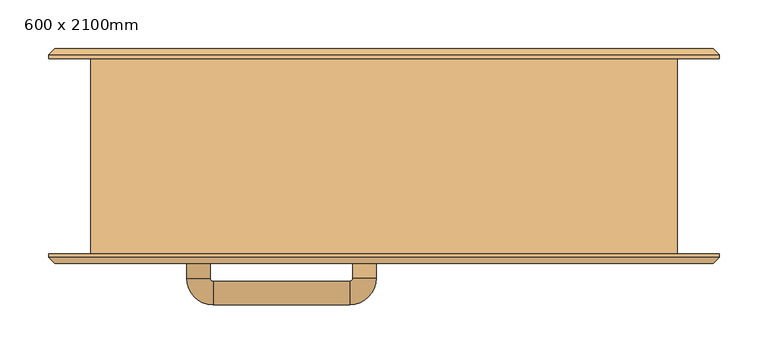
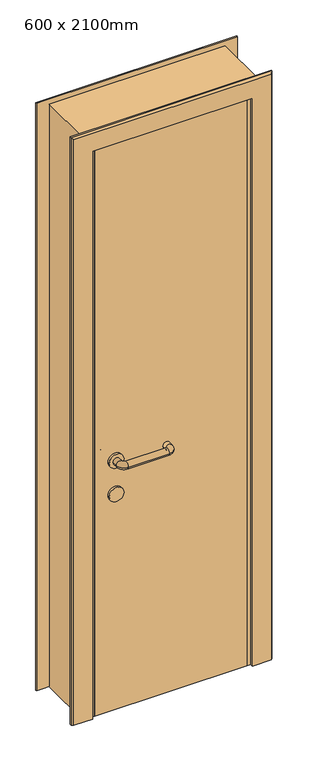
"""IFC4 building model written with IfcOpenShell, lengths in millimetres: door geometry, Porta única com revestimento : 600 x 2100mm."""

from ifc_helpers import new_model, si_unit, point, frame, frame_2d, origin, origin_with_axes, place, context, project, spatial, polyline, circle_curve, ellipse_curve, trimmed, segment, composite_curve, outline, extrude, faceted_brep, source, transform, mapped, element, save
from ifc_brep_helpers import plane_surface, cylinder_surface, revolved_surface, advanced_brep


def door_600_x_2100mm_c47176d9(model_context):
    return source(origin(), model_context, "Body", "SolidModel", [
        advanced_brep(
        [(-178.0, -57.0, 900.0), (-202.0, -57.0, 900.0), (-178.0, -40.0, 900.0), (-202.0, -40.0, 900.0), (-175.0, -13.0, 900.0), (-175.0, -37.0, 900.0), (-35.0, -37.0, 900.0), (-35.0, -13.0, 900.0), (-8.0, -40.0, 900.0), (-32.0, -40.0, 900.0), (-32.0, -55.0, 900.0), (-8.0, -55.0, 900.0)],
        [
            (0, 1, circle_curve(frame((-190.0, -57.0, 900.0), z_axis=(0.0, -1.0, 0.0), x_axis=(-1.0, 0.0, 0.0)), 12.0)),
            (1, 0, circle_curve(frame((-190.0, -57.0, 900.0), z_axis=(0.0, -1.0, 0.0), x_axis=(-1.0, 0.0, 0.0)), 12.0)),
            (0, 2),
            (2, 3, circle_curve(frame((-190.0, -40.0, 900.0), z_axis=(0.0, -1.0, 0.0), x_axis=(-1.0, 0.0, 0.0)), 12.0)),
            (3, 1),
            (3, 2, circle_curve(frame((-190.0, -40.0, 900.0), z_axis=(0.0, -1.0, 0.0), x_axis=(-1.0, 0.0, 0.0)), 12.0)),
            (4, 3, circle_curve(frame((-175.0, -40.0, 900.0), z_axis=(0.0, 0.0, 1.0), x_axis=(-1.0, 0.0, 0.0)), 27.0)),
            (2, 5, circle_curve(frame((-175.0, -40.0, 900.0), z_axis=(0.0, 0.0, -1.0), x_axis=(-1.0, 0.0, 0.0)), 3.0)),
            (5, 4, circle_curve(frame((-175.0, -25.0, 900.0), z_axis=(-1.0, 0.0, 0.0), x_axis=(0.0, 1.0, 0.0)), 12.0)),
            (4, 5, circle_curve(frame((-175.0, -25.0, 900.0), z_axis=(-1.0, 0.0, 0.0), x_axis=(0.0, 1.0, 0.0)), 12.0)),
            (5, 6),
            (6, 7, circle_curve(frame((-35.0, -25.0, 900.0), z_axis=(-1.0, 0.0, 0.0), x_axis=(0.0, 1.0, 0.0)), 12.0)),
            (7, 4),
            (7, 6, circle_curve(frame((-35.0, -25.0, 900.0), z_axis=(-1.0, 0.0, 0.0), x_axis=(0.0, 1.0, 0.0)), 12.0)),
            (8, 7, circle_curve(frame((-35.0, -40.0, 900.0), z_axis=(0.0, 0.0, 1.0), x_axis=(0.0, 1.0, 0.0)), 27.0)),
            (6, 9, circle_curve(frame((-35.0, -40.0, 900.0), z_axis=(0.0, 0.0, -1.0), x_axis=(0.0, 1.0, 0.0)), 3.0)),
            (9, 8, circle_curve(frame((-20.0, -40.0, 900.0), z_axis=(0.0, 1.0, 0.0), x_axis=(1.0, 0.0, 0.0)), 12.0)),
            (8, 9, circle_curve(frame((-20.0, -40.0, 900.0), z_axis=(0.0, 1.0, 0.0), x_axis=(1.0, 0.0, 0.0)), 12.0)),
            (10, 11, circle_curve(frame((-20.0, -55.0, 900.0), z_axis=(0.0, -1.0, 0.0), x_axis=(1.0, 0.0, 0.0)), 12.0)),
            (11, 10, circle_curve(frame((-20.0, -55.0, 900.0), z_axis=(0.0, -1.0, 0.0), x_axis=(1.0, 0.0, 0.0)), 12.0)),
            (9, 10),
            (11, 8),
        ],
        [
            plane_surface(frame((-1032.0, -57.0, 1730.0), z_axis=(0.0, -1.0, 0.0), x_axis=(0.0, 0.0, 1.0))),
            cylinder_surface(frame((-190.0, -57.0, 900.0), z_axis=(0.0, -1.0, 0.0), x_axis=(-1.0, 0.0, 0.0)), 12.0),
            revolved_surface(trimmed(ellipse_curve(frame((-190.0, -40.0, 900.0), z_axis=(0.0, -1.0, 0.0), x_axis=(-1.0, 0.0, 0.0)), 12.0, 12.0), [point((-178.0, -40.0, 900.0))], [point((-202.0, -40.0, 900.0))], True, "CARTESIAN"), (-175.0, -40.0, 1730.0), (0.0, 0.0, -1.0)),
            revolved_surface(trimmed(ellipse_curve(frame((-190.0, -40.0, 900.0), z_axis=(0.0, -1.0, 0.0), x_axis=(-1.0, 0.0, 0.0)), 12.0, 12.0), [point((-202.0, -40.0, 900.0))], [point((-178.0, -40.0, 900.0))], True, "CARTESIAN"), (-175.0, -40.0, 1730.0), (0.0, 0.0, -1.0)),
            cylinder_surface(frame((-175.0, -25.0, 900.0), z_axis=(-1.0, 0.0, 0.0), x_axis=(0.0, 1.0, 0.0)), 12.0),
            revolved_surface(trimmed(ellipse_curve(frame((-35.0, -25.0, 900.0), z_axis=(-1.0, 0.0, 0.0), x_axis=(0.0, 1.0, 0.0)), 12.0, 12.0), [point((-35.0, -37.0, 900.0))], [point((-35.0, -13.0, 900.0))], True, "CARTESIAN"), (-35.0, -40.0, 1730.0), (0.0, 0.0, -1.0)),
            revolved_surface(trimmed(ellipse_curve(frame((-35.0, -25.0, 900.0), z_axis=(-1.0, 0.0, 0.0), x_axis=(0.0, 1.0, 0.0)), 12.0, 12.0), [point((-35.0, -13.0, 900.0))], [point((-35.0, -37.0, 900.0))], True, "CARTESIAN"), (-35.0, -40.0, 1730.0), (0.0, 0.0, -1.0)),
            plane_surface(frame((-862.0, -55.0, 1730.0), z_axis=(0.0, -1.0, 0.0), x_axis=(0.0, 0.0, -1.0))),
            cylinder_surface(frame((-20.0, -40.0, 900.0), z_axis=(0.0, 1.0, 0.0), x_axis=(1.0, 0.0, 0.0)), 12.0),
        ],
        [
            (0, [[1, 2]]),
            (1, [[-1, 3, 4, 5]]),
            (1, [[-2, -5, 6, -3]]),
            (2, [[7, -4, 8, 9]]),
            (3, [[-8, -6, -7, 10]]),
            (4, [[-9, 11, 12, 13]]),
            (4, [[-10, -13, 14, -11]]),
            (5, [[15, -12, 16, 17]]),
            (6, [[-16, -14, -15, 18]]),
            (7, [[19, 20]]),
            (8, [[-17, 21, -20, 22]]),
            (8, [[-18, -22, -19, -21]]),
        ],
    ),
        extrude(outline(composite_curve([segment(trimmed(circle_curve(frame_2d((780.0, -190.0)), 25.0), [point((780.0, -215.0))], [point((780.0, -165.0))], False, "CARTESIAN"), True, "CONTINUOUS"), segment(trimmed(circle_curve(frame_2d((780.0, -190.0)), 25.0), [point((780.0, -165.0))], [point((780.0, -215.0))], False, "CARTESIAN"), True, "CONTINUOUS")], self_intersect=False)), frame((0.0, -65.0, 0.0), z_axis=(0.0, 1.0, 0.0), x_axis=(0.0, 0.0, 1.0)), (0.0, 0.0, 1.0), 8.0),
        extrude(outline(composite_curve([segment(trimmed(circle_curve(frame_2d((900.0, -190.0)), 25.0), [point((900.0, -215.0))], [point((900.0, -165.0))], False, "CARTESIAN"), True, "CONTINUOUS"), segment(trimmed(circle_curve(frame_2d((900.0, -190.0)), 25.0), [point((900.0, -165.0))], [point((900.0, -215.0))], False, "CARTESIAN"), True, "CONTINUOUS")], self_intersect=False)), frame((0.0, -65.0, 0.0), z_axis=(0.0, 1.0, 0.0), x_axis=(0.0, 0.0, 1.0)), (0.0, 0.0, 1.0), 8.0),
        advanced_brep(
        [(-202.0, -108.0, 900.0), (-178.0, -108.0, 900.0), (-202.0, -125.0, 900.0), (-178.0, -125.0, 900.0), (-175.0, -128.0, 900.0), (-175.0, -152.0, 900.0), (-35.0, -152.0, 900.0), (-35.0, -128.0, 900.0), (-32.0, -125.0, 900.0), (-8.0, -125.0, 900.0), (-8.0, -110.0, 900.0), (-32.0, -110.0, 900.0)],
        [
            (0, 1, circle_curve(frame((-190.0, -108.0, 900.0), z_axis=(0.0, 1.0, 0.0), x_axis=(1.0, 0.0, 0.0)), 12.0)),
            (1, 0, circle_curve(frame((-190.0, -108.0, 900.0), z_axis=(0.0, 1.0, 0.0), x_axis=(1.0, 0.0, 0.0)), 12.0)),
            (0, 2),
            (2, 3, circle_curve(frame((-190.0, -125.0, 900.0), z_axis=(0.0, 1.0, 0.0), x_axis=(1.0, 0.0, 0.0)), 12.0)),
            (3, 1),
            (3, 2, circle_curve(frame((-190.0, -125.0, 900.0), z_axis=(0.0, 1.0, 0.0), x_axis=(1.0, 0.0, 0.0)), 12.0)),
            (4, 3, circle_curve(frame((-175.0, -125.0, 900.0), z_axis=(0.0, 0.0, -1.0), x_axis=(-1.0, 0.0, 0.0)), 3.0)),
            (2, 5, circle_curve(frame((-175.0, -125.0, 900.0), z_axis=(0.0, 0.0, 1.0), x_axis=(-1.0, 0.0, 0.0)), 27.0)),
            (5, 4, circle_curve(frame((-175.0, -140.0, 900.0), z_axis=(-1.0, 0.0, 0.0), x_axis=(0.0, 1.0, 0.0)), 12.0)),
            (4, 5, circle_curve(frame((-175.0, -140.0, 900.0), z_axis=(-1.0, 0.0, 0.0), x_axis=(0.0, 1.0, 0.0)), 12.0)),
            (5, 6),
            (6, 7, circle_curve(frame((-35.0, -140.0, 900.0), z_axis=(-1.0, 0.0, 0.0), x_axis=(0.0, 1.0, 0.0)), 12.0)),
            (7, 4),
            (7, 6, circle_curve(frame((-35.0, -140.0, 900.0), z_axis=(-1.0, 0.0, 0.0), x_axis=(0.0, 1.0, 0.0)), 12.0)),
            (8, 7, circle_curve(frame((-35.0, -125.0, 900.0), z_axis=(0.0, 0.0, -1.0), x_axis=(0.0, -1.0, 0.0)), 3.0)),
            (6, 9, circle_curve(frame((-35.0, -125.0, 900.0), z_axis=(0.0, 0.0, 1.0), x_axis=(0.0, -1.0, 0.0)), 27.0)),
            (9, 8, circle_curve(frame((-20.0, -125.0, 900.0), z_axis=(0.0, -1.0, 0.0), x_axis=(-1.0, 0.0, 0.0)), 12.0)),
            (8, 9, circle_curve(frame((-20.0, -125.0, 900.0), z_axis=(0.0, -1.0, 0.0), x_axis=(-1.0, 0.0, 0.0)), 12.0)),
            (10, 11, circle_curve(frame((-20.0, -110.0, 900.0), z_axis=(0.0, 1.0, 0.0), x_axis=(-1.0, 0.0, 0.0)), 12.0)),
            (11, 10, circle_curve(frame((-20.0, -110.0, 900.0), z_axis=(0.0, 1.0, 0.0), x_axis=(-1.0, 0.0, 0.0)), 12.0)),
            (9, 10),
            (11, 8),
        ],
        [
            plane_surface(frame((-1032.0, -108.0, 1730.0), z_axis=(0.0, 1.0, 0.0), x_axis=(0.0, 0.0, -1.0))),
            cylinder_surface(frame((-190.0, -108.0, 900.0), z_axis=(0.0, 1.0, 0.0), x_axis=(1.0, 0.0, 0.0)), 12.0),
            revolved_surface(trimmed(ellipse_curve(frame((-190.0, -125.0, 900.0), z_axis=(0.0, 1.0, 0.0), x_axis=(1.0, 0.0, 0.0)), 12.0, 12.0), [point((-202.0, -125.0, 900.0))], [point((-178.0, -125.0, 900.0))], True, "CARTESIAN"), (-175.0, -125.0, 1730.0), (0.0, 0.0, 1.0)),
            revolved_surface(trimmed(ellipse_curve(frame((-190.0, -125.0, 900.0), z_axis=(0.0, 1.0, 0.0), x_axis=(1.0, 0.0, 0.0)), 12.0, 12.0), [point((-178.0, -125.0, 900.0))], [point((-202.0, -125.0, 900.0))], True, "CARTESIAN"), (-175.0, -125.0, 1730.0), (0.0, 0.0, 1.0)),
            cylinder_surface(frame((-175.0, -140.0, 900.0), z_axis=(-1.0, 0.0, 0.0), x_axis=(0.0, 1.0, 0.0)), 12.0),
            revolved_surface(trimmed(ellipse_curve(frame((-35.0, -140.0, 900.0), z_axis=(-1.0, 0.0, 0.0), x_axis=(0.0, 1.0, 0.0)), 12.0, 12.0), [point((-35.0, -152.0, 900.0))], [point((-35.0, -128.0, 900.0))], True, "CARTESIAN"), (-35.0, -125.0, 1730.0), (0.0, 0.0, 1.0)),
            revolved_surface(trimmed(ellipse_curve(frame((-35.0, -140.0, 900.0), z_axis=(-1.0, 0.0, 0.0), x_axis=(0.0, 1.0, 0.0)), 12.0, 12.0), [point((-35.0, -128.0, 900.0))], [point((-35.0, -152.0, 900.0))], True, "CARTESIAN"), (-35.0, -125.0, 1730.0), (0.0, 0.0, 1.0)),
            plane_surface(frame((-862.0, -110.0, 1730.0), z_axis=(0.0, 1.0, 0.0), x_axis=(0.0, 0.0, 1.0))),
            cylinder_surface(frame((-20.0, -125.0, 900.0), z_axis=(0.0, -1.0, 0.0), x_axis=(-1.0, 0.0, 0.0)), 12.0),
        ],
        [
            (0, [[1, 2]]),
            (1, [[-1, 3, 4, 5]]),
            (1, [[-2, -5, 6, -3]]),
            (2, [[7, -4, 8, 9]]),
            (3, [[-8, -6, -7, 10]]),
            (4, [[-9, 11, 12, 13]]),
            (4, [[-10, -13, 14, -11]]),
            (5, [[15, -12, 16, 17]]),
            (6, [[-16, -14, -15, 18]]),
            (7, [[19, 20]]),
            (8, [[-17, 21, -20, 22]]),
            (8, [[-18, -22, -19, -21]]),
        ],
    ),
        extrude(outline(composite_curve([segment(trimmed(circle_curve(frame_2d((780.0, -190.0)), 25.0), [point((780.0, -215.0))], [point((780.0, -165.0))], False, "CARTESIAN"), True, "CONTINUOUS"), segment(trimmed(circle_curve(frame_2d((780.0, -190.0)), 25.0), [point((780.0, -165.0))], [point((780.0, -215.0))], False, "CARTESIAN"), True, "CONTINUOUS")], self_intersect=False)), frame((0.0, -108.0, 0.0), z_axis=(0.0, 1.0, 0.0), x_axis=(0.0, 0.0, 1.0)), (0.0, 0.0, 1.0), 8.0),
        extrude(outline(composite_curve([segment(trimmed(circle_curve(frame_2d((900.0, -190.0)), 25.0), [point((900.0, -215.0))], [point((900.0, -165.0))], False, "CARTESIAN"), True, "CONTINUOUS"), segment(trimmed(circle_curve(frame_2d((900.0, -190.0)), 25.0), [point((900.0, -165.0))], [point((900.0, -215.0))], False, "CARTESIAN"), True, "CONTINUOUS")], self_intersect=False)), frame((0.0, -108.0, 0.0), z_axis=(0.0, 1.0, 0.0), x_axis=(0.0, 0.0, 1.0)), (0.0, 0.0, 1.0), 8.0),
        extrude(outline(polyline([(260.0, -65.0), (260.0, -100.0), (-260.0, -100.0), (-260.0, -65.0), (260.0, -65.0)])), origin_with_axes(), (0.0, 0.0, 1.0), 2060.0),
        faceted_brep([(343.0, 104.0, 0.0), (343.0, 100.0, 0.0), (273.0, 100.0, 0.0), (273.0, 110.0, 0.0), (337.0, 110.0, 0.0), (343.0, 104.0, 2118.0), (343.0, 100.0, 2118.0), (-343.0, 100.0, 2118.0), (-343.0, 100.0, 0.0), (-273.0, 100.0, 0.0), (-273.0, 100.0, 2048.0), (273.0, 100.0, 2048.0), (273.0, 110.0, 2048.0), (-273.0, 110.0, 2048.0), (-273.0, 110.0, 0.0), (-337.0, 110.0, 0.0), (-337.0, 110.0, 2112.0), (337.0, 110.0, 2112.0), (-343.0, 104.0, 0.0), (-343.0, 104.0, 2118.0)], [[[0, 1, 2, 3, 4]], [[1, 0, 5, 6]], [[2, 1, 6, 7, 8, 9, 10, 11]], [[3, 2, 11, 12]], [[4, 3, 12, 13, 14, 15, 16, 17]], [[0, 4, 17, 5]], [[18, 15, 14, 9, 8]], [[19, 16, 15, 18]], [[13, 10, 9, 14]], [[7, 19, 18, 8]], [[5, 17, 16, 19]], [[12, 11, 10, 13]], [[6, 5, 19, 7]]]),
        faceted_brep([(343.0, -104.0, 0.0), (337.0, -110.0, 0.0), (273.0, -110.0, 0.0), (273.0, -100.0, 0.0), (343.0, -100.0, 0.0), (343.0, -104.0, 2118.0), (337.0, -110.0, 2112.0), (-337.0, -110.0, 2112.0), (-337.0, -110.0, 0.0), (-273.0, -110.0, 0.0), (-273.0, -110.0, 2048.0), (273.0, -110.0, 2048.0), (273.0, -100.0, 2048.0), (-273.0, -100.0, 2048.0), (-273.0, -100.0, 0.0), (-343.0, -100.0, 0.0), (-343.0, -100.0, 2118.0), (343.0, -100.0, 2118.0), (-343.0, -104.0, 2118.0), (-343.0, -104.0, 0.0)], [[[0, 1, 2, 3, 4]], [[1, 0, 5, 6]], [[2, 1, 6, 7, 8, 9, 10, 11]], [[3, 2, 11, 12]], [[4, 3, 12, 13, 14, 15, 16, 17]], [[0, 4, 17, 5]], [[7, 18, 19, 8]], [[19, 15, 14, 9, 8]], [[13, 10, 9, 14]], [[18, 16, 15, 19]], [[6, 5, 18, 7]], [[12, 11, 10, 13]], [[5, 17, 16, 18]]]),
        faceted_brep([(300.0, 100.0, 0.0), (300.0, -100.0, 0.0), (260.0, -100.0, 0.0), (260.0, -65.0, 0.0), (250.0, -65.0, 0.0), (250.0, 100.0, 0.0), (300.0, 100.0, 2100.0), (300.0, -100.0, 2100.0), (-300.0, -100.0, 2100.0), (-300.0, -100.0, 0.0), (-260.0, -100.0, 0.0), (-260.0, -100.0, 2060.0), (260.0, -100.0, 2060.0), (260.0, -65.0, 2060.0), (-260.0, -65.0, 2060.0), (-260.0, -65.0, 0.0), (-250.0, -65.0, 0.0), (-250.0, -65.0, 2050.0), (250.0, -65.0, 2050.0), (250.0, 100.0, 2050.0), (-250.0, 100.0, 2050.0), (-250.0, 100.0, 0.0), (-300.0, 100.0, 0.0), (-300.0, 100.0, 2100.0)], [[[0, 1, 2, 3, 4, 5]], [[1, 0, 6, 7]], [[2, 1, 7, 8, 9, 10, 11, 12]], [[3, 2, 12, 13]], [[4, 3, 13, 14, 15, 16, 17, 18]], [[5, 4, 18, 19]], [[0, 5, 19, 20, 21, 22, 23, 6]], [[8, 23, 22, 9]], [[22, 21, 16, 15, 10, 9]], [[14, 11, 10, 15]], [[20, 17, 16, 21]], [[7, 6, 23, 8]], [[13, 12, 11, 14]], [[19, 18, 17, 20]]]),
    ])


if __name__ == "__main__":
    model = new_model("IFC4")
    model_context = context("Model", 3, world=origin())
    ifc_project = project(units=[si_unit("LENGTHUNIT", "METRE", prefix="MILLI")], contexts=[model_context])
    site = spatial("IfcSite", under=ifc_project)
    building = spatial("IfcBuilding", under=site)
    placement = place(None, origin())
    door_600_x_2100mm_shape = door_600_x_2100mm_c47176d9(model_context)
    element("IfcDoor", 1, ObjectType="Porta única com revestimento : 600 x 2100mm", at=placement, inside=building, context=model_context, shape_type="MappedRepresentation", body=[
        mapped(door_600_x_2100mm_shape, transform((0.0, 0.0, 0.0), x_axis=(1.0, 0.0, 0.0), y_axis=(0.0, 1.0, 0.0), z_axis=(0.0, 0.0, 1.0))),
    ])
    save(model, "model.ifc")

# Revit data of these elements
# Type "Porta única com revestimento : 600 x 2100mm"
#   Type Mark = "31"
#   Construction Type Id = "MDOOR"
#   Analytic Construction = "Metal"
#   Largura da apara = 70 mm
#   Espessura da apara = 10 mm
#   Thickness = 35 mm
#   Rough Width = 600 mm
#   Rough Height = 2100 mm
#   Heat Transfer Coefficient (U) = 3.7021 W/(m²·K)
#   Height = 2100 mm
#   Width = 600 mm
#   Largura da moldura média = 40 mm
#   Largura da estrutura = 50 mm
#   Material da apara = none
#   Material do painel = none
#   Material do puxador = none
#   Material da moldura = none
#   Visual Light Transmittance = 0
#   Solar Heat Gain Coefficient = 0
#   Function = (empty or 0)
#   Wall Closure = (empty or 0)
